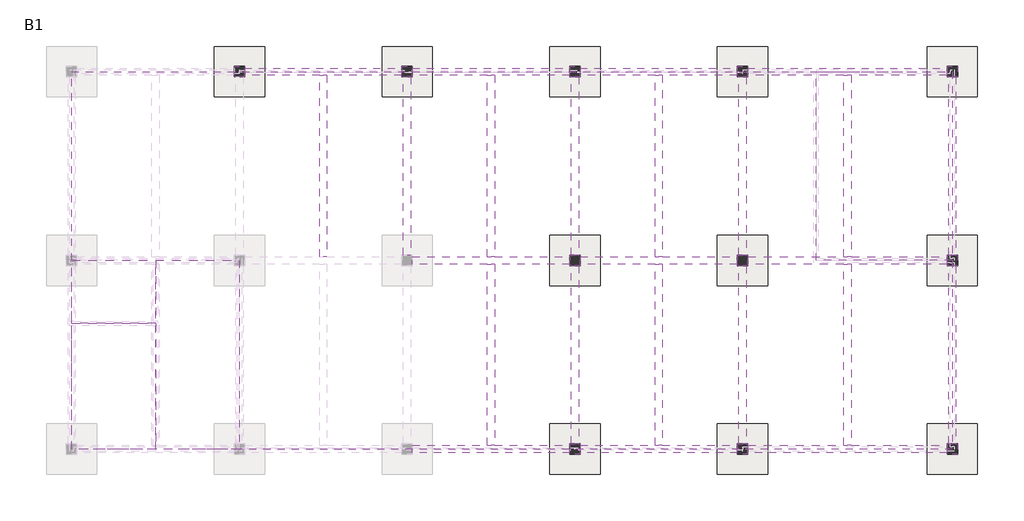
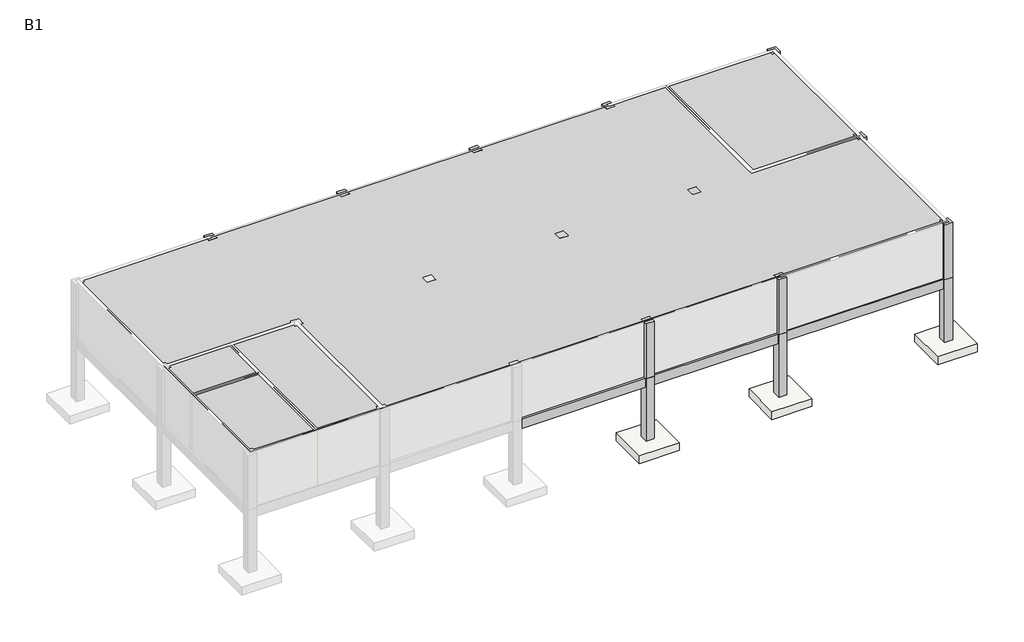
# One storey, part 2 of 2: 24 beams, 22 columns, 11 slabs, 5 proxies.
"""IFC4 building model written with IfcOpenShell, lengths in millimetres."""

import ifcopenshell
import ifcopenshell.guid

model = None  # the IFC model being written
_history = None  # IfcOwnerHistory: only IFC2X3 demands one
_inside = {}  # id of a spatial element -> (the spatial element, [elements in it])
_under = {}  # id of a project, library or spatial element -> (it, [spatial elements below it])
_declared = {}  # id of a project -> (the project, [libraries it declares])
_typed = {}  # id of a type object -> (the type object, [elements of that type])
_made_of = {}  # id of a material, layer set ... -> (it, [elements and type objects made of it])


def new_model(schema):
    """Start an empty IFC model of exactly this schema.

    Asked for "IFC4X3", IfcOpenShell would pick the latest addendum, in which some entities
    have other attributes; the version numbers below select the first issue.
    IFC2X3 requires an IfcOwnerHistory on every rooted entity: one is made here for all.
    """
    global model, _history
    if schema == "IFC4X3":
        model = ifcopenshell.file(schema_version=(4, 3, 0, 0))
    else:
        model = ifcopenshell.file(schema=schema)
    _inside.clear()
    _under.clear()
    _declared.clear()
    _typed.clear()
    _made_of.clear()
    _history = None
    if model.schema == "IFC2X3":
        org = make("IfcOrganization", Name="unknown")
        user = make(
            "IfcPersonAndOrganization",
            ThePerson=make("IfcPerson", FamilyName="unknown"),
            TheOrganization=org,
        )
        app = make(
            "IfcApplication",
            ApplicationDeveloper=org,
            Version="unknown",
            ApplicationFullName="unknown",
            ApplicationIdentifier="unknown",
        )
        _history = make(
            "IfcOwnerHistory",
            OwningUser=user,
            OwningApplication=app,
            ChangeAction="ADDED",
            CreationDate=0,
        )
    return model


def make(cls, **values):
    """One entity of the class cls with the attributes given. An attribute that is None is left unset."""
    return model.create_entity(
        cls, **{name: value for name, value in values.items() if value is not None}
    )


def rooted(cls, **values):
    """An entity with a GlobalId (a new one), such as an element, a storey or a relation."""
    return make(cls, GlobalId=ifcopenshell.guid.new(), OwnerHistory=_history, **values)


def si_unit(unit_type, name, prefix=None):
    """IfcSIUnit, for example si_unit("LENGTHUNIT", "METRE", prefix="MILLI")."""
    return make("IfcSIUnit", UnitType=unit_type, Prefix=prefix, Name=name)


def assignment(units):
    """IfcUnitAssignment: the units of a project."""
    return None if units is None else make("IfcUnitAssignment", Units=units)


def point(xyz):
    """IfcCartesianPoint."""
    return None if xyz is None else make("IfcCartesianPoint", Coordinates=xyz)


def direction(xyz):
    """IfcDirection."""
    return None if xyz is None else make("IfcDirection", DirectionRatios=xyz)


def frame(location, z_axis=None, x_axis=None):
    """IfcAxis2Placement3D, a coordinate frame: its origin and axes. An axis left out is left unset."""
    return make(
        "IfcAxis2Placement3D",
        Location=point(location),
        Axis=direction(z_axis),
        RefDirection=direction(x_axis),
    )


def origin():
    """The frame at (0, 0, 0) with its axes left unset."""
    return frame((0.0, 0.0, 0.0))


def origin_with_axes():
    """The frame at (0, 0, 0) with the z axis (0, 0, 1) and the x axis (1, 0, 0) written out."""
    return frame((0.0, 0.0, 0.0), z_axis=(0.0, 0.0, 1.0), x_axis=(1.0, 0.0, 0.0))


def place(relative_to, where):
    """IfcLocalPlacement: puts the frame where relative to a parent placement (None: the world)."""
    return make(
        "IfcLocalPlacement", PlacementRelTo=relative_to, RelativePlacement=where
    )


def context(
    kind, dimensions, precision=None, world=None, true_north=None, identifier=None
):
    """IfcGeometricRepresentationContext, for example the 3D "Model" context."""
    return make(
        "IfcGeometricRepresentationContext",
        ContextIdentifier=identifier,
        ContextType=kind,
        CoordinateSpaceDimension=dimensions,
        Precision=precision,
        WorldCoordinateSystem=world,
        TrueNorth=true_north,
    )


def project(units=None, contexts=None):
    """IfcProject with its units and contexts."""
    return rooted(
        "IfcProject",
        Name="project",
        RepresentationContexts=contexts,
        UnitsInContext=assignment(units),
    )


def spatial(cls, under=None, at=None, **own):
    """A site, building, storey or space (cls), placed at a placement, below another one or the project."""
    s = rooted(cls, ObjectPlacement=at, **own)
    if under is not None:
        _under.setdefault(under.id(), (under, []))[1].append(s)
    return s


def polyline(points):
    """IfcPolyline through the points."""
    return make("IfcPolyline", Points=[point(p) for p in points])


def outline(outer, holes=None, kind="AREA"):
    """IfcArbitraryClosedProfileDef: a profile drawn as a closed curve; with holes, ...WithVoids."""
    if holes is None:
        return make("IfcArbitraryClosedProfileDef", ProfileType=kind, OuterCurve=outer)
    return make(
        "IfcArbitraryProfileDefWithVoids",
        ProfileType=kind,
        OuterCurve=outer,
        InnerCurves=holes,
    )


def extrude(swept, where, along, depth):
    """IfcExtrudedAreaSolid: the profile swept, set in the frame where, extruded along a direction by depth."""
    return make(
        "IfcExtrudedAreaSolid",
        SweptArea=swept,
        Position=where,
        ExtrudedDirection=direction(along),
        Depth=depth,
    )


def faces_of(points, faces, orient=None, outer=None):
    """IfcFace entities. A face is a list of loops; a loop is a list of indices into points, from 0.

    orient and outer hold one flag for each loop. By default every Orientation is true, the
    first loop of a face is its IfcFaceOuterBound and the others are IfcFaceBound.
    """
    made = []
    for i, loops in enumerate(faces):
        bounds = []
        for j, loop in enumerate(loops):
            is_outer = j == 0 if outer is None else outer[i][j]
            bounds.append(
                make(
                    "IfcFaceOuterBound" if is_outer else "IfcFaceBound",
                    Bound=make("IfcPolyLoop", Polygon=[points[k] for k in loop]),
                    Orientation=True if orient is None else orient[i][j],
                )
            )
        made.append(make("IfcFace", Bounds=bounds))
    return made


def faceted_brep(points, faces, orient=None, outer=None, voids=None):
    """IfcFacetedBrep: a solid bounded by flat faces; with voids (closed shells), ...WithVoids."""
    shared = [point(p) for p in points]
    hull = make("IfcClosedShell", CfsFaces=faces_of(shared, faces, orient, outer))
    if voids is None:
        return make("IfcFacetedBrep", Outer=hull)
    return make(
        "IfcFacetedBrepWithVoids",
        Outer=hull,
        Voids=[
            make(cls, CfsFaces=faces_of(shared, fs, o, b)) for cls, fs, o, b in voids
        ],
    )


def shape(context_of_items, identifier, shape_type, items):
    """IfcShapeRepresentation: the items that make up one representation, for example the "Body"."""
    return make(
        "IfcShapeRepresentation",
        ContextOfItems=context_of_items,
        RepresentationIdentifier=identifier,
        RepresentationType=shape_type,
        Items=items,
    )


def source(mapping_origin, context_of_items, identifier, shape_type, items):
    """IfcRepresentationMap: a shape defined once, which mapped items show again and again."""
    return make(
        "IfcRepresentationMap",
        MappingOrigin=mapping_origin,
        MappedRepresentation=shape(context_of_items, identifier, shape_type, items),
    )


def transform(
    local_origin,
    x_axis=None,
    y_axis=None,
    z_axis=None,
    scale=None,
    scale2=None,
    scale3=None,
    uniform=True,
):
    """IfcCartesianTransformationOperator3D, or its non-uniform kind. x_axis, y_axis, z_axis: its Axis1, 2, 3."""
    if uniform:
        return make(
            "IfcCartesianTransformationOperator3D",
            Axis1=direction(x_axis),
            Axis2=direction(y_axis),
            LocalOrigin=point(local_origin),
            Scale=scale,
            Axis3=direction(z_axis),
        )
    return make(
        "IfcCartesianTransformationOperator3DnonUniform",
        Axis1=direction(x_axis),
        Axis2=direction(y_axis),
        LocalOrigin=point(local_origin),
        Scale=scale,
        Axis3=direction(z_axis),
        Scale2=scale2,
        Scale3=scale3,
    )


def mapped(mapping_source, mapping_target):
    """IfcMappedItem: shows the shape of a source again, moved by a transform."""
    return make(
        "IfcMappedItem", MappingSource=mapping_source, MappingTarget=mapping_target
    )


def made_of(thing, what):
    """Note that an element or type object is made of a material, layer set ...; save() writes the relation."""
    if what is not None:
        _made_of.setdefault(what.id(), (what, []))[1].append(thing)
    return thing


def element(
    cls,
    number,
    at=None,
    inside=None,
    cuts=None,
    type_object=None,
    material=None,
    context=None,
    identifier="Body",
    shape_type=None,
    held_by="IfcProductDefinitionShape",
    body=None,
    shapes=None,
    **own,
):
    """One element of the class cls, such as IfcWall. Its Tag is "e" and its number.

    at: its placement. inside: the storey or other place that contains it. cuts: it is an
    opening in that element (IfcRelVoidsElement). A single representation is given by context,
    identifier, shape_type and body (its items); several are given by shapes. held_by: the class
    of the entity that holds the representations. save() writes the other relations.
    """
    e = rooted(cls, Tag="e%d" % number, ObjectPlacement=at, **own)
    if body is not None:
        shapes = [shape(context, identifier, shape_type, body)]
    if shapes is not None:
        e.Representation = make(held_by, Representations=shapes)
    if inside is not None:
        _inside.setdefault(inside.id(), (inside, []))[1].append(e)
    if cuts is not None:
        rooted(
            "IfcRelVoidsElement", RelatingBuildingElement=cuts, RelatedOpeningElement=e
        )
    if type_object is not None:
        _typed.setdefault(type_object.id(), (type_object, []))[1].append(e)
    return made_of(e, material)


def aggregate(whole, parts):
    """IfcRelAggregates: a whole, such as a stair, and the parts it consists of."""
    return rooted("IfcRelAggregates", RelatingObject=whole, RelatedObjects=parts)


def save(model, path):
    """Write the relations noted so far, then the file.

    IfcRelAggregates (storeys below a building ...), IfcRelContainedInSpatialStructure (elements
    in a storey), IfcRelDefinesByType, IfcRelAssociatesMaterial and IfcRelDeclares: one each for
    every whole, place, type object, material and project.
    """
    for whole, parts in _under.values():
        aggregate(whole, parts)
    for where, things in _inside.values():
        rooted(
            "IfcRelContainedInSpatialStructure",
            RelatedElements=things,
            RelatingStructure=where,
        )
    for kind, things in _typed.values():
        rooted("IfcRelDefinesByType", RelatedObjects=things, RelatingType=kind)
    for what, things in _made_of.values():
        rooted("IfcRelAssociatesMaterial", RelatedObjects=things, RelatingMaterial=what)
    for by, libraries in _declared.values():
        rooted("IfcRelDeclares", RelatingContext=by, RelatedDefinitions=libraries)
    model.write(path)


def generic_models_bb515c93(model_context):
    return source(origin(), model_context, "Body", "SweptSolid", [
        extrude(outline(polyline([(9000.0, 21000.0), (9000.0, -21000.0), (-9000.0, -21000.0), (-9000.0, 21000.0), (9000.0, 21000.0)])), origin_with_axes(), (0.0, 0.0, 1.0), 3500.0),
    ])


def generic_models_5926095e(model_context):
    return source(origin(), model_context, "Body", "SweptSolid", [
        extrude(outline(polyline([(3250.0, 4500.0), (3250.0, -4500.0), (-3250.0, -4500.0), (-3250.0, 4500.0), (3250.0, 4500.0)])), origin_with_axes(), (0.0, 0.0, 1.0), 3500.0),
    ])


def generic_models_0b067365(model_context):
    return source(origin(), model_context, "Body", "SweptSolid", [
        extrude(outline(polyline([(2000.0, 4500.0), (2000.0, -4500.0), (-2000.0, -4500.0), (-2000.0, 4500.0), (2000.0, 4500.0)])), origin_with_axes(), (0.0, 0.0, 1.0), 3500.0),
    ])


def generic_models_4c644d41(model_context):
    return source(origin(), model_context, "Body", "SweptSolid", [
        extrude(outline(polyline([(2000.0, 1500.0), (2000.0, -1500.0), (-2000.0, -1500.0), (-2000.0, 1500.0), (2000.0, 1500.0)])), origin_with_axes(), (0.0, 0.0, 1.0), 3500.0),
    ])


def generic_models_c89eb543(model_context):
    return source(origin(), model_context, "Body", "SweptSolid", [
        extrude(outline(polyline([(2000.0, 3000.0), (2000.0, -3000.0), (-2000.0, -3000.0), (-2000.0, 3000.0), (2000.0, 3000.0)])), origin_with_axes(), (0.0, 0.0, 1.0), 3500.0),
    ])


def ft112_footing_rectangular_ft112_2400x2400x500_5fe39465(model_context):
    return source(origin(), model_context, "Body", "SweptSolid", [
        extrude(outline(polyline([(1200.0, 1200.0), (1200.0, -1200.0), (-1200.0, -1200.0), (-1200.0, 1200.0), (1200.0, 1200.0)])), frame((0.0, 0.0, -500.0), z_axis=(0.0, 0.0, 1.0), x_axis=(1.0, 0.0, 0.0)), (0.0, 0.0, 1.0), 500.0),
    ])


model = new_model("IFC4")

# Units and contexts
model_context = context("Model", 3, world=origin())
ifc_project = project(units=[si_unit("LENGTHUNIT", "METRE", prefix="MILLI")], contexts=[model_context])

# Site, building, storey
site = spatial("IfcSite", under=ifc_project)
building = spatial("IfcBuilding", under=site)
storey = spatial("IfcBuildingStorey", under=building, Name="B1", Elevation=-4000.0)

# Beams
placement = place(None, origin())
element("IfcBeam", 1, ObjectType="Concrete-Rectangular-Beam : BM111_400x500_RG1", at=placement, inside=storey, context=model_context, shape_type="SweptSolid", body=[
    extrude(outline(polyline([(57634.6521483, 173098.8614395), (57284.6521483, 173098.8614395), (57284.6521483, 181748.8614395), (57634.6521483, 181748.8614395), (57634.6521483, 173098.8614395)])), frame((0.0, 0.0, -600.0), z_axis=(0.0, 0.0, 1.0), x_axis=(1.0, 0.0, 0.0)), (0.0, 0.0, 1.0), 600.0),
])
element("IfcBeam", 2, ObjectType="Concrete-Rectangular-Beam : BM111_400x500_RG1", at=placement, inside=storey, context=model_context, shape_type="SweptSolid", body=[
    extrude(outline(polyline([(65634.6521483, 173098.8614395), (65284.6521483, 173098.8614395), (65284.6521483, 181748.8614395), (65634.6521483, 181748.8614395), (65634.6521483, 173098.8614395)])), frame((0.0, 0.0, -600.0), z_axis=(0.0, 0.0, 1.0), x_axis=(1.0, 0.0, 0.0)), (0.0, 0.0, 1.0), 600.0),
])
element("IfcBeam", 3, ObjectType="Concrete-Rectangular-Beam : BM111_400x500_RG1", at=placement, inside=storey, context=model_context, shape_type="SweptSolid", body=[
    extrude(outline(polyline([(65284.6521483, 172748.8614395), (65634.6521483, 172748.8614395), (65634.6521483, 164098.8614395), (65284.6521483, 164098.8614395), (65284.6521483, 172748.8614395)])), frame((0.0, 0.0, -600.0), z_axis=(0.0, 0.0, 1.0), x_axis=(1.0, 0.0, 0.0)), (0.0, 0.0, 1.0), 600.0),
])
element("IfcBeam", 4, ObjectType="Concrete-Rectangular-Beam : BM111_400x500_RG1", at=placement, inside=storey, context=model_context, shape_type="SweptSolid", body=[
    extrude(outline(polyline([(73634.6521483, 173098.8614395), (73284.6521483, 173098.8614395), (73284.6521483, 181748.8614395), (73634.6521483, 181748.8614395), (73634.6521483, 173098.8614395)])), frame((0.0, 0.0, -600.0), z_axis=(0.0, 0.0, 1.0), x_axis=(1.0, 0.0, 0.0)), (0.0, 0.0, 1.0), 600.0),
])
element("IfcBeam", 5, ObjectType="Concrete-Rectangular-Beam : BM111_400x500_RG1", at=placement, inside=storey, context=model_context, shape_type="SweptSolid", body=[
    extrude(outline(polyline([(73284.6521483, 172748.8614395), (73634.6521483, 172748.8614395), (73634.6521483, 164098.8614395), (73284.6521483, 164098.8614395), (73284.6521483, 172748.8614395)])), frame((0.0, 0.0, -600.0), z_axis=(0.0, 0.0, 1.0), x_axis=(1.0, 0.0, 0.0)), (0.0, 0.0, 1.0), 600.0),
])
element("IfcBeam", 6, ObjectType="Concrete-Rectangular-Beam : BM111_400x500_RG1", at=placement, inside=storey, context=model_context, shape_type="SweptSolid", body=[
    extrude(outline(polyline([(82634.6521483, 173098.8614395), (82284.6521483, 173098.8614395), (82284.6521483, 181748.8614395), (82634.6521483, 181748.8614395), (82634.6521483, 173098.8614395)])), frame((0.0, 0.0, -600.0), z_axis=(0.0, 0.0, 1.0), x_axis=(1.0, 0.0, 0.0)), (0.0, 0.0, 1.0), 600.0),
])
element("IfcBeam", 7, ObjectType="Concrete-Rectangular-Beam : BM111_400x500_RG1", at=placement, inside=storey, context=model_context, shape_type="SweptSolid", body=[
    extrude(outline(polyline([(82284.6521483, 172748.8614395), (82634.6521483, 172748.8614395), (82634.6521483, 164098.8614395), (82284.6521483, 164098.8614395), (82284.6521483, 172748.8614395)])), frame((0.0, 0.0, -600.0), z_axis=(0.0, 0.0, 1.0), x_axis=(1.0, 0.0, 0.0)), (0.0, 0.0, 1.0), 600.0),
])
element("IfcBeam", 8, ObjectType="Concrete-Rectangular-Beam : BM111_400x500_RG1", at=placement, inside=storey, context=model_context, shape_type="Brep", body=[
    faceted_brep([(53709.6521483, 182098.8614395, 0.0), (53709.6521483, 181748.8614395, 0.0), (57284.6521483, 181748.8614395, 0.0), (57634.6521483, 181748.8614395, 0.0), (61209.6521483, 181748.8614395, 0.0), (61209.6521483, 182098.8614395, 0.0), (53709.6521483, 181748.8614395, -600.0), (57284.6521483, 181748.8614395, -600.0), (57634.6521483, 181748.8614395, -600.0), (61209.6521483, 181748.8614395, -600.0), (53709.6521483, 182098.8614395, -600.0), (61209.6521483, 182098.8614395, -600.0)], [[[0, 1, 2, 3, 4, 5]], [[1, 6, 7, 8, 9, 4, 3, 2]], [[6, 10, 11, 9, 8, 7]], [[10, 0, 5, 11]], [[1, 0, 10, 6]], [[5, 4, 9, 11]]]),
])
element("IfcBeam", 9, ObjectType="Concrete-Rectangular-Beam : BM111_400x500_RG1", at=placement, inside=storey, context=model_context, shape_type="Brep", body=[
    faceted_brep([(61709.6521483, 182098.8614395, 0.0), (61709.6521483, 181748.8614395, 0.0), (65284.6521483, 181748.8614395, 0.0), (65634.6521483, 181748.8614395, 0.0), (69209.6521483, 181748.8614395, 0.0), (69209.6521483, 182098.8614395, 0.0), (61709.6521483, 181748.8614395, -600.0), (65284.6521483, 181748.8614395, -600.0), (65634.6521483, 181748.8614395, -600.0), (69209.6521483, 181748.8614395, -600.0), (61709.6521483, 182098.8614395, -600.0), (69209.6521483, 182098.8614395, -600.0)], [[[0, 1, 2, 3, 4, 5]], [[1, 6, 7, 8, 9, 4, 3, 2]], [[6, 10, 11, 9, 8, 7]], [[10, 0, 5, 11]], [[1, 0, 10, 6]], [[5, 4, 9, 11]]]),
])
element("IfcBeam", 10, ObjectType="Concrete-Rectangular-Beam : BM111_400x500_RG1", at=placement, inside=storey, context=model_context, shape_type="Brep", body=[
    faceted_brep([(69709.6521483, 182098.8614395, 0.0), (69709.6521483, 181748.8614395, 0.0), (73284.6521483, 181748.8614395, 0.0), (73634.6521483, 181748.8614395, 0.0), (77209.6521483, 181748.8614395, 0.0), (77209.6521483, 182098.8614395, 0.0), (69709.6521483, 181748.8614395, -600.0), (73284.6521483, 181748.8614395, -600.0), (73634.6521483, 181748.8614395, -600.0), (77209.6521483, 181748.8614395, -600.0), (69709.6521483, 182098.8614395, -600.0), (77209.6521483, 182098.8614395, -600.0)], [[[0, 1, 2, 3, 4, 5]], [[1, 6, 7, 8, 9, 4, 3, 2]], [[6, 10, 11, 9, 8, 7]], [[10, 0, 5, 11]], [[1, 0, 10, 6]], [[5, 4, 9, 11]]]),
])
element("IfcBeam", 11, ObjectType="Concrete-Rectangular-Beam : BM111_400x500_RG1", at=placement, inside=storey, context=model_context, shape_type="Brep", body=[
    faceted_brep([(77709.6521483, 182098.8614395, 0.0), (77709.6521483, 181748.8614395, 0.0), (82284.6521483, 181748.8614395, 0.0), (82634.6521483, 181748.8614395, 0.0), (87209.6521483, 181748.8614395, 0.0), (87209.6521483, 182098.8614395, 0.0), (77709.6521483, 181748.8614395, -600.0), (82284.6521483, 181748.8614395, -600.0), (82634.6521483, 181748.8614395, -600.0), (87209.6521483, 181748.8614395, -600.0), (77709.6521483, 182098.8614395, -600.0), (87209.6521483, 182098.8614395, -600.0)], [[[0, 1, 2, 3, 4, 5]], [[1, 6, 7, 8, 9, 4, 3, 2]], [[6, 10, 11, 9, 8, 7]], [[10, 0, 5, 11]], [[1, 0, 10, 6]], [[5, 4, 9, 11]]]),
])
element("IfcBeam", 12, ObjectType="Concrete-Rectangular-Beam : BM111_400x500_RG1", at=placement, inside=storey, context=model_context, shape_type="Brep", body=[
    faceted_brep([(61709.6521483, 173098.8614395, 0.0), (61709.6521483, 172748.8614395, 0.0), (65284.6521483, 172748.8614395, 0.0), (65634.6521483, 172748.8614395, 0.0), (69209.6521483, 172748.8614395, 0.0), (69209.6521483, 173098.8614395, 0.0), (65634.6521483, 173098.8614395, 0.0), (65284.6521483, 173098.8614395, 0.0), (61709.6521483, 172748.8614395, -600.0), (65284.6521483, 172748.8614395, -600.0), (65634.6521483, 172748.8614395, -600.0), (69209.6521483, 172748.8614395, -600.0), (61709.6521483, 173098.8614395, -600.0), (65284.6521483, 173098.8614395, -600.0), (65634.6521483, 173098.8614395, -600.0), (69209.6521483, 173098.8614395, -600.0)], [[[0, 1, 2, 3, 4, 5, 6, 7]], [[1, 8, 9, 10, 11, 4, 3, 2]], [[8, 12, 13, 14, 15, 11, 10, 9]], [[12, 0, 7, 6, 5, 15, 14, 13]], [[1, 0, 12, 8]], [[5, 4, 11, 15]]]),
])
element("IfcBeam", 13, ObjectType="Concrete-Rectangular-Beam : BM111_400x500_RG1", at=placement, inside=storey, context=model_context, shape_type="Brep", body=[
    faceted_brep([(69709.6521483, 173098.8614395, 0.0), (69709.6521483, 172748.8614395, 0.0), (73284.6521483, 172748.8614395, 0.0), (73634.6521483, 172748.8614395, 0.0), (77209.6521483, 172748.8614395, 0.0), (77209.6521483, 173098.8614395, 0.0), (73634.6521483, 173098.8614395, 0.0), (73284.6521483, 173098.8614395, 0.0), (69709.6521483, 172748.8614395, -600.0), (73284.6521483, 172748.8614395, -600.0), (73634.6521483, 172748.8614395, -600.0), (77209.6521483, 172748.8614395, -600.0), (69709.6521483, 173098.8614395, -600.0), (73284.6521483, 173098.8614395, -600.0), (73634.6521483, 173098.8614395, -600.0), (77209.6521483, 173098.8614395, -600.0)], [[[0, 1, 2, 3, 4, 5, 6, 7]], [[1, 8, 9, 10, 11, 4, 3, 2]], [[8, 12, 13, 14, 15, 11, 10, 9]], [[12, 0, 7, 6, 5, 15, 14, 13]], [[1, 0, 12, 8]], [[5, 4, 11, 15]]]),
])
element("IfcBeam", 14, ObjectType="Concrete-Rectangular-Beam : BM111_400x500_RG1", at=placement, inside=storey, context=model_context, shape_type="Brep", body=[
    faceted_brep([(77709.6521483, 173098.8614395, 0.0), (77709.6521483, 172748.8614395, 0.0), (82284.6521483, 172748.8614395, 0.0), (82634.6521483, 172748.8614395, 0.0), (87209.6521483, 172748.8614395, 0.0), (87209.6521483, 173098.8614395, 0.0), (82634.6521483, 173098.8614395, 0.0), (82284.6521483, 173098.8614395, 0.0), (77709.6521483, 172748.8614395, -600.0), (82284.6521483, 172748.8614395, -600.0), (82634.6521483, 172748.8614395, -600.0), (87209.6521483, 172748.8614395, -600.0), (77709.6521483, 173098.8614395, -600.0), (82284.6521483, 173098.8614395, -600.0), (82634.6521483, 173098.8614395, -600.0), (87209.6521483, 173098.8614395, -600.0)], [[[0, 1, 2, 3, 4, 5, 6, 7]], [[1, 8, 9, 10, 11, 4, 3, 2]], [[8, 12, 13, 14, 15, 11, 10, 9]], [[12, 0, 7, 6, 5, 15, 14, 13]], [[1, 0, 12, 8]], [[5, 4, 11, 15]]]),
])
element("IfcBeam", 15, ObjectType="Concrete-Rectangular-Beam : BM111_400x500_RG1", at=placement, inside=storey, context=model_context, shape_type="Brep", body=[
    faceted_brep([(61709.6521483, 164098.8614395, 0.0), (61709.6521483, 163748.8614395, 0.0), (69209.6521483, 163748.8614395, 0.0), (69209.6521483, 164098.8614395, 0.0), (65634.6521483, 164098.8614395, 0.0), (65284.6521483, 164098.8614395, 0.0), (61709.6521483, 163748.8614395, -600.0), (69209.6521483, 163748.8614395, -600.0), (61709.6521483, 164098.8614395, -600.0), (65284.6521483, 164098.8614395, -600.0), (65634.6521483, 164098.8614395, -600.0), (69209.6521483, 164098.8614395, -600.0)], [[[0, 1, 2, 3, 4, 5]], [[1, 6, 7, 2]], [[6, 8, 9, 10, 11, 7]], [[8, 0, 5, 4, 3, 11, 10, 9]], [[1, 0, 8, 6]], [[3, 2, 7, 11]]]),
])
element("IfcBeam", 16, ObjectType="Concrete-Rectangular-Beam : BM111_400x500_RG1", at=placement, inside=storey, context=model_context, shape_type="Brep", body=[
    faceted_brep([(69709.6521483, 164098.8614395, 0.0), (69709.6521483, 163748.8614395, 0.0), (77209.6521483, 163748.8614395, 0.0), (77209.6521483, 164098.8614395, 0.0), (73634.6521483, 164098.8614395, 0.0), (73284.6521483, 164098.8614395, 0.0), (69709.6521483, 163748.8614395, -600.0), (77209.6521483, 163748.8614395, -600.0), (69709.6521483, 164098.8614395, -600.0), (73284.6521483, 164098.8614395, -600.0), (73634.6521483, 164098.8614395, -600.0), (77209.6521483, 164098.8614395, -600.0)], [[[0, 1, 2, 3, 4, 5]], [[1, 6, 7, 2]], [[6, 8, 9, 10, 11, 7]], [[8, 0, 5, 4, 3, 11, 10, 9]], [[1, 0, 8, 6]], [[3, 2, 7, 11]]]),
])
element("IfcBeam", 17, ObjectType="Concrete-Rectangular-Beam : BM111_400x500_RG1", at=placement, inside=storey, context=model_context, shape_type="Brep", body=[
    faceted_brep([(77709.6521483, 164098.8614395, 0.0), (77709.6521483, 163748.8614395, 0.0), (87209.6521483, 163748.8614395, 0.0), (87209.6521483, 164098.8614395, 0.0), (82634.6521483, 164098.8614395, 0.0), (82284.6521483, 164098.8614395, 0.0), (77709.6521483, 163748.8614395, -600.0), (87209.6521483, 163748.8614395, -600.0), (77709.6521483, 164098.8614395, -600.0), (82284.6521483, 164098.8614395, -600.0), (82634.6521483, 164098.8614395, -600.0), (87209.6521483, 164098.8614395, -600.0)], [[[0, 1, 2, 3, 4, 5]], [[1, 6, 7, 2]], [[6, 8, 9, 10, 11, 7]], [[8, 0, 5, 4, 3, 11, 10, 9]], [[1, 0, 8, 6]], [[3, 2, 7, 11]]]),
])
element("IfcBeam", 18, ObjectType="Concrete-Rectangular-Beam : BM111_400x500_RG1", at=placement, inside=storey, context=model_context, shape_type="SweptSolid", body=[
    extrude(outline(polyline([(61284.6521483, 181673.8614395), (61634.6521483, 181673.8614395), (61634.6521483, 173173.8614395), (61284.6521483, 173173.8614395), (61284.6521483, 181673.8614395)])), frame((0.0, 0.0, -600.0), z_axis=(0.0, 0.0, 1.0), x_axis=(1.0, 0.0, 0.0)), (0.0, 0.0, 1.0), 600.0),
])
element("IfcBeam", 19, ObjectType="Concrete-Rectangular-Beam : BM111_400x500_RG1", at=placement, inside=storey, context=model_context, shape_type="SweptSolid", body=[
    extrude(outline(polyline([(69284.6521483, 181673.8614395), (69634.6521483, 181673.8614395), (69634.6521483, 173173.8614395), (69284.6521483, 173173.8614395), (69284.6521483, 181673.8614395)])), frame((0.0, 0.0, -600.0), z_axis=(0.0, 0.0, 1.0), x_axis=(1.0, 0.0, 0.0)), (0.0, 0.0, 1.0), 600.0),
])
element("IfcBeam", 20, ObjectType="Concrete-Rectangular-Beam : BM111_400x500_RG1", at=placement, inside=storey, context=model_context, shape_type="SweptSolid", body=[
    extrude(outline(polyline([(69284.6521483, 172673.8614395), (69634.6521483, 172673.8614395), (69634.6521483, 164173.8614395), (69284.6521483, 164173.8614395), (69284.6521483, 172673.8614395)])), frame((0.0, 0.0, -600.0), z_axis=(0.0, 0.0, 1.0), x_axis=(1.0, 0.0, 0.0)), (0.0, 0.0, 1.0), 600.0),
])
element("IfcBeam", 21, ObjectType="Concrete-Rectangular-Beam : BM111_400x500_RG1", at=placement, inside=storey, context=model_context, shape_type="SweptSolid", body=[
    extrude(outline(polyline([(77284.6521483, 181673.8614395), (77634.6521483, 181673.8614395), (77634.6521483, 173173.8614395), (77284.6521483, 173173.8614395), (77284.6521483, 181673.8614395)])), frame((0.0, 0.0, -600.0), z_axis=(0.0, 0.0, 1.0), x_axis=(1.0, 0.0, 0.0)), (0.0, 0.0, 1.0), 600.0),
])
element("IfcBeam", 22, ObjectType="Concrete-Rectangular-Beam : BM111_400x500_RG1", at=placement, inside=storey, context=model_context, shape_type="SweptSolid", body=[
    extrude(outline(polyline([(77284.6521483, 172673.8614395), (77634.6521483, 172673.8614395), (77634.6521483, 164173.8614395), (77284.6521483, 164173.8614395), (77284.6521483, 172673.8614395)])), frame((0.0, 0.0, -600.0), z_axis=(0.0, 0.0, 1.0), x_axis=(1.0, 0.0, 0.0)), (0.0, 0.0, 1.0), 600.0),
])
element("IfcBeam", 23, ObjectType="Concrete-Rectangular-Beam : BM111_400x500_RG1", at=placement, inside=storey, context=model_context, shape_type="SweptSolid", body=[
    extrude(outline(polyline([(87284.6521483, 181673.8614395), (87634.6521483, 181673.8614395), (87634.6521483, 173173.8614395), (87284.6521483, 173173.8614395), (87284.6521483, 181673.8614395)])), frame((0.0, 0.0, -600.0), z_axis=(0.0, 0.0, 1.0), x_axis=(1.0, 0.0, 0.0)), (0.0, 0.0, 1.0), 600.0),
])
element("IfcBeam", 24, ObjectType="Concrete-Rectangular-Beam : BM111_400x500_RG1", at=placement, inside=storey, context=model_context, shape_type="SweptSolid", body=[
    extrude(outline(polyline([(87284.6521483, 172673.8614395), (87634.6521483, 172673.8614395), (87634.6521483, 164173.8614395), (87284.6521483, 164173.8614395), (87284.6521483, 172673.8614395)])), frame((0.0, 0.0, -600.0), z_axis=(0.0, 0.0, 1.0), x_axis=(1.0, 0.0, 0.0)), (0.0, 0.0, 1.0), 600.0),
])

# Proxies
generic_models_shape = generic_models_bb515c93(model_context)
element("IfcBuildingElementProxy", 25, Name="Space Planning Box_hec : Space Planning Box_hec", ObjectType="Space Planning Box_hec : Space Planning Box_hec", at=placement, inside=storey, context=model_context, shape_type="MappedRepresentation", body=[
    mapped(generic_models_shape, transform((66459.6521483, 172923.8614395, 0.0), x_axis=(0.0, -1.0, 0.0), y_axis=(1.0, 0.0, 0.0), z_axis=(0.0, 0.0, 1.0))),
])
generic_models_2_shape = generic_models_5926095e(model_context)
element("IfcBuildingElementProxy", 26, Name="Space Planning Box_hec : Space Planning Box_hec", ObjectType="Space Planning Box_hec : Space Planning Box_hec", at=placement, inside=storey, context=model_context, shape_type="MappedRepresentation", body=[
    mapped(generic_models_2_shape, transform((84209.6521483, 177423.8614395, 0.0), x_axis=(1.0, 0.0, 0.0), y_axis=(0.0, 1.0, 0.0), z_axis=(0.0, 0.0, 1.0))),
])
generic_models_3_shape = generic_models_0b067365(model_context)
element("IfcBuildingElementProxy", 27, Name="Space Planning Box_hec : Space Planning Box_hec", ObjectType="Space Planning Box_hec : Space Planning Box_hec", at=placement, inside=storey, context=model_context, shape_type="MappedRepresentation", body=[
    mapped(generic_models_3_shape, transform((51459.6521483, 168423.8614395, 0.0), x_axis=(1.0, 0.0, 0.0), y_axis=(0.0, 1.0, 0.0), z_axis=(0.0, 0.0, 1.0))),
])
generic_models_4_shape = generic_models_4c644d41(model_context)
element("IfcBuildingElementProxy", 28, Name="Space Planning Box_hec : Space Planning Box_hec", ObjectType="Space Planning Box_hec : Space Planning Box_hec", at=placement, inside=storey, context=model_context, shape_type="MappedRepresentation", body=[
    mapped(generic_models_4_shape, transform((47459.6521483, 171423.8614395, 0.0), x_axis=(1.0, 0.0, 0.0), y_axis=(0.0, 1.0, 0.0), z_axis=(0.0, 0.0, 1.0))),
])
generic_models_5_shape = generic_models_c89eb543(model_context)
element("IfcBuildingElementProxy", 29, Name="Space Planning Box_hec : Space Planning Box_hec", ObjectType="Space Planning Box_hec : Space Planning Box_hec", at=placement, inside=storey, context=model_context, shape_type="MappedRepresentation", body=[
    mapped(generic_models_5_shape, transform((47459.6521483, 166923.8614395, 0.0), x_axis=(1.0, 0.0, 0.0), y_axis=(0.0, 1.0, 0.0), z_axis=(0.0, 0.0, 1.0))),
])

# Columns
element("IfcColumn", 30, ObjectType="Concrete-Rectangular-Column : CL111_500x500", at=placement, inside=storey, context=model_context, shape_type="Brep", body=[
    faceted_brep([(53709.6521483, 182173.8614395, 0.0), (53709.6521483, 181673.8614395, 0.0), (53209.6521483, 181673.8614395, 0.0), (53209.6521483, 182173.8614395, 0.0), (53709.6521483, 182173.8614395, 3500.0), (53709.6521483, 182098.8614395, 3500.0), (53709.6521483, 181748.8614395, 3500.0), (53709.6521483, 181673.8614395, 3500.0), (53634.6521483, 181673.8614395, 3500.0), (53284.6521483, 181673.8614395, 3500.0), (53209.6521483, 181673.8614395, 3500.0), (53209.6521483, 181748.8614395, 3500.0), (53209.6521483, 182098.8614395, 3500.0), (53209.6521483, 182173.8614395, 3500.0)], [[[0, 1, 2, 3]], [[4, 5, 6, 7, 1, 0]], [[7, 8, 9, 10, 2, 1]], [[10, 11, 12, 13, 3, 2]], [[13, 4, 0, 3]], [[4, 13, 12, 11, 10, 9, 8, 7, 6, 5]]]),
])
element("IfcColumn", 31, ObjectType="Concrete-Rectangular-Column : CL111_500x500", at=placement, inside=storey, context=model_context, shape_type="Brep", body=[
    faceted_brep([(61709.6521483, 182173.8614395, 0.0), (61709.6521483, 181673.8614395, 0.0), (61209.6521483, 181673.8614395, 0.0), (61209.6521483, 182173.8614395, 0.0), (61709.6521483, 182173.8614395, 3500.0), (61709.6521483, 182098.8614395, 3500.0), (61709.6521483, 181748.8614395, 3500.0), (61709.6521483, 181673.8614395, 3500.0), (61634.6521483, 181673.8614395, 3500.0), (61284.6521483, 181673.8614395, 3500.0), (61209.6521483, 181673.8614395, 3500.0), (61209.6521483, 181748.8614395, 3500.0), (61209.6521483, 182098.8614395, 3500.0), (61209.6521483, 182173.8614395, 3500.0)], [[[0, 1, 2, 3]], [[4, 5, 6, 7, 1, 0]], [[7, 8, 9, 10, 2, 1]], [[10, 11, 12, 13, 3, 2]], [[13, 4, 0, 3]], [[4, 13, 12, 11, 10, 9, 8, 7, 6, 5]]]),
])
element("IfcColumn", 32, ObjectType="Concrete-Rectangular-Column : CL111_500x500", at=placement, inside=storey, context=model_context, shape_type="Brep", body=[
    faceted_brep([(69709.6521483, 182173.8614395, 0.0), (69709.6521483, 181673.8614395, 0.0), (69209.6521483, 181673.8614395, 0.0), (69209.6521483, 182173.8614395, 0.0), (69709.6521483, 182173.8614395, 3500.0), (69709.6521483, 182098.8614395, 3500.0), (69709.6521483, 181748.8614395, 3500.0), (69709.6521483, 181673.8614395, 3500.0), (69634.6521483, 181673.8614395, 3500.0), (69284.6521483, 181673.8614395, 3500.0), (69209.6521483, 181673.8614395, 3500.0), (69209.6521483, 181748.8614395, 3500.0), (69209.6521483, 182098.8614395, 3500.0), (69209.6521483, 182173.8614395, 3500.0)], [[[0, 1, 2, 3]], [[4, 5, 6, 7, 1, 0]], [[7, 8, 9, 10, 2, 1]], [[10, 11, 12, 13, 3, 2]], [[13, 4, 0, 3]], [[4, 13, 12, 11, 10, 9, 8, 7, 6, 5]]]),
])
element("IfcColumn", 33, ObjectType="Concrete-Rectangular-Column : CL111_500x500", at=placement, inside=storey, context=model_context, shape_type="Brep", body=[
    faceted_brep([(77709.6521483, 182173.8614395, 0.0), (77709.6521483, 181673.8614395, 0.0), (77209.6521483, 181673.8614395, 0.0), (77209.6521483, 182173.8614395, 0.0), (77709.6521483, 182173.8614395, 3500.0), (77709.6521483, 182098.8614395, 3500.0), (77709.6521483, 181748.8614395, 3500.0), (77709.6521483, 181673.8614395, 3500.0), (77634.6521483, 181673.8614395, 3500.0), (77284.6521483, 181673.8614395, 3500.0), (77209.6521483, 181673.8614395, 3500.0), (77209.6521483, 181748.8614395, 3500.0), (77209.6521483, 182098.8614395, 3500.0), (77209.6521483, 182173.8614395, 3500.0)], [[[0, 1, 2, 3]], [[4, 5, 6, 7, 1, 0]], [[7, 8, 9, 10, 2, 1]], [[10, 11, 12, 13, 3, 2]], [[13, 4, 0, 3]], [[4, 13, 12, 11, 10, 9, 8, 7, 6, 5]]]),
])
element("IfcColumn", 34, ObjectType="Concrete-Rectangular-Column : CL111_500x500", at=placement, inside=storey, context=model_context, shape_type="Brep", body=[
    faceted_brep([(87709.6521483, 182173.8614395, 0.0), (87709.6521483, 181673.8614395, 0.0), (87209.6521483, 181673.8614395, 0.0), (87209.6521483, 182173.8614395, 0.0), (87709.6521483, 182173.8614395, 3500.0), (87709.6521483, 181673.8614395, 3500.0), (87634.6521483, 181673.8614395, 3500.0), (87284.6521483, 181673.8614395, 3500.0), (87209.6521483, 181673.8614395, 3500.0), (87209.6521483, 181748.8614395, 3500.0), (87209.6521483, 182098.8614395, 3500.0), (87209.6521483, 182173.8614395, 3500.0)], [[[0, 1, 2, 3]], [[4, 5, 1, 0]], [[5, 6, 7, 8, 2, 1]], [[8, 9, 10, 11, 3, 2]], [[11, 4, 0, 3]], [[4, 11, 10, 9, 8, 7, 6, 5]]]),
])
element("IfcColumn", 35, ObjectType="Concrete-Rectangular-Column : CL111_500x500", at=placement, inside=storey, context=model_context, shape_type="Brep", body=[
    faceted_brep([(69709.6521483, 173173.8614395, 0.0), (69709.6521483, 172673.8614395, 0.0), (69209.6521483, 172673.8614395, 0.0), (69209.6521483, 173173.8614395, 0.0), (69709.6521483, 173173.8614395, 3500.0), (69709.6521483, 173098.8614395, 3500.0), (69709.6521483, 172748.8614395, 3500.0), (69709.6521483, 172673.8614395, 3500.0), (69634.6521483, 172673.8614395, 3500.0), (69284.6521483, 172673.8614395, 3500.0), (69209.6521483, 172673.8614395, 3500.0), (69209.6521483, 172748.8614395, 3500.0), (69209.6521483, 173098.8614395, 3500.0), (69209.6521483, 173173.8614395, 3500.0), (69284.6521483, 173173.8614395, 3500.0), (69634.6521483, 173173.8614395, 3500.0)], [[[0, 1, 2, 3]], [[4, 5, 6, 7, 1, 0]], [[7, 8, 9, 10, 2, 1]], [[10, 11, 12, 13, 3, 2]], [[13, 14, 15, 4, 0, 3]], [[4, 15, 14, 13, 12, 11, 10, 9, 8, 7, 6, 5]]]),
])
element("IfcColumn", 36, ObjectType="Concrete-Rectangular-Column : CL111_500x500", at=placement, inside=storey, context=model_context, shape_type="Brep", body=[
    faceted_brep([(77709.6521483, 173173.8614395, 0.0), (77709.6521483, 172673.8614395, 0.0), (77209.6521483, 172673.8614395, 0.0), (77209.6521483, 173173.8614395, 0.0), (77709.6521483, 173173.8614395, 3500.0), (77709.6521483, 173098.8614395, 3500.0), (77709.6521483, 172748.8614395, 3500.0), (77709.6521483, 172673.8614395, 3500.0), (77634.6521483, 172673.8614395, 3500.0), (77284.6521483, 172673.8614395, 3500.0), (77209.6521483, 172673.8614395, 3500.0), (77209.6521483, 172748.8614395, 3500.0), (77209.6521483, 173098.8614395, 3500.0), (77209.6521483, 173173.8614395, 3500.0), (77284.6521483, 173173.8614395, 3500.0), (77634.6521483, 173173.8614395, 3500.0)], [[[0, 1, 2, 3]], [[4, 5, 6, 7, 1, 0]], [[7, 8, 9, 10, 2, 1]], [[10, 11, 12, 13, 3, 2]], [[13, 14, 15, 4, 0, 3]], [[4, 15, 14, 13, 12, 11, 10, 9, 8, 7, 6, 5]]]),
])
element("IfcColumn", 37, ObjectType="Concrete-Rectangular-Column : CL111_500x500", at=placement, inside=storey, context=model_context, shape_type="Brep", body=[
    faceted_brep([(87709.6521483, 173173.8614395, 0.0), (87709.6521483, 172673.8614395, 0.0), (87209.6521483, 172673.8614395, 0.0), (87209.6521483, 173173.8614395, 0.0), (87709.6521483, 173173.8614395, 3500.0), (87709.6521483, 172673.8614395, 3500.0), (87634.6521483, 172673.8614395, 3500.0), (87284.6521483, 172673.8614395, 3500.0), (87209.6521483, 172673.8614395, 3500.0), (87209.6521483, 172748.8614395, 3500.0), (87209.6521483, 173098.8614395, 3500.0), (87209.6521483, 173173.8614395, 3500.0), (87284.6521483, 173173.8614395, 3500.0), (87634.6521483, 173173.8614395, 3500.0)], [[[0, 1, 2, 3]], [[4, 5, 1, 0]], [[5, 6, 7, 8, 2, 1]], [[8, 9, 10, 11, 3, 2]], [[11, 12, 13, 4, 0, 3]], [[4, 13, 12, 11, 10, 9, 8, 7, 6, 5]]]),
])
element("IfcColumn", 38, ObjectType="Concrete-Rectangular-Column : CL111_500x500", at=placement, inside=storey, context=model_context, shape_type="Brep", body=[
    faceted_brep([(69709.6521483, 164173.8614395, 0.0), (69709.6521483, 163673.8614395, 0.0), (69209.6521483, 163673.8614395, 0.0), (69209.6521483, 164173.8614395, 0.0), (69709.6521483, 164173.8614395, 3500.0), (69709.6521483, 164098.8614395, 3500.0), (69709.6521483, 163748.8614395, 3500.0), (69709.6521483, 163673.8614395, 3500.0), (69209.6521483, 163673.8614395, 3500.0), (69209.6521483, 163748.8614395, 3500.0), (69209.6521483, 164098.8614395, 3500.0), (69209.6521483, 164173.8614395, 3500.0), (69284.6521483, 164173.8614395, 3500.0), (69634.6521483, 164173.8614395, 3500.0)], [[[0, 1, 2, 3]], [[4, 5, 6, 7, 1, 0]], [[7, 8, 2, 1]], [[8, 9, 10, 11, 3, 2]], [[11, 12, 13, 4, 0, 3]], [[4, 13, 12, 11, 10, 9, 8, 7, 6, 5]]]),
])
element("IfcColumn", 39, ObjectType="Concrete-Rectangular-Column : CL111_500x500", at=placement, inside=storey, context=model_context, shape_type="Brep", body=[
    faceted_brep([(77709.6521483, 164173.8614395, 0.0), (77709.6521483, 163673.8614395, 0.0), (77209.6521483, 163673.8614395, 0.0), (77209.6521483, 164173.8614395, 0.0), (77709.6521483, 164173.8614395, 3500.0), (77709.6521483, 164098.8614395, 3500.0), (77709.6521483, 163748.8614395, 3500.0), (77709.6521483, 163673.8614395, 3500.0), (77209.6521483, 163673.8614395, 3500.0), (77209.6521483, 163748.8614395, 3500.0), (77209.6521483, 164098.8614395, 3500.0), (77209.6521483, 164173.8614395, 3500.0), (77284.6521483, 164173.8614395, 3500.0), (77634.6521483, 164173.8614395, 3500.0)], [[[0, 1, 2, 3]], [[4, 5, 6, 7, 1, 0]], [[7, 8, 2, 1]], [[8, 9, 10, 11, 3, 2]], [[11, 12, 13, 4, 0, 3]], [[4, 13, 12, 11, 10, 9, 8, 7, 6, 5]]]),
])
element("IfcColumn", 40, ObjectType="Concrete-Rectangular-Column : CL111_500x500", at=placement, inside=storey, context=model_context, shape_type="Brep", body=[
    faceted_brep([(87709.6521483, 164173.8614395, 0.0), (87709.6521483, 163673.8614395, 0.0), (87209.6521483, 163673.8614395, 0.0), (87209.6521483, 164173.8614395, 0.0), (87709.6521483, 164173.8614395, 3500.0), (87709.6521483, 163673.8614395, 3500.0), (87209.6521483, 163673.8614395, 3500.0), (87209.6521483, 163748.8614395, 3500.0), (87209.6521483, 164098.8614395, 3500.0), (87209.6521483, 164173.8614395, 3500.0), (87284.6521483, 164173.8614395, 3500.0), (87634.6521483, 164173.8614395, 3500.0)], [[[0, 1, 2, 3]], [[4, 5, 1, 0]], [[5, 6, 2, 1]], [[6, 7, 8, 9, 3, 2]], [[9, 10, 11, 4, 0, 3]], [[4, 11, 10, 9, 8, 7, 6, 5]]]),
])
element("IfcColumn", 41, ObjectType="Concrete-Rectangular-Column : CL111_500x500", at=placement, inside=storey, context=model_context, shape_type="Brep", body=[
    faceted_brep([(53709.6521483, 182173.8614395, -4000.0), (53709.6521483, 181673.8614395, -4000.0), (53209.6521483, 181673.8614395, -4000.0), (53209.6521483, 182173.8614395, -4000.0), (53709.6521483, 182173.8614395, 0.0), (53709.6521483, 182098.8614395, 0.0), (53709.6521483, 181748.8614395, 0.0), (53709.6521483, 181673.8614395, 0.0), (53634.6521483, 181673.8614395, 0.0), (53284.6521483, 181673.8614395, 0.0), (53209.6521483, 181673.8614395, 0.0), (53209.6521483, 181748.8614395, 0.0), (53209.6521483, 182098.8614395, 0.0), (53209.6521483, 182173.8614395, 0.0)], [[[0, 1, 2, 3]], [[4, 5, 6, 7, 1, 0]], [[7, 8, 9, 10, 2, 1]], [[10, 11, 12, 13, 3, 2]], [[13, 4, 0, 3]], [[4, 13, 12, 11, 10, 9, 8, 7, 6, 5]]]),
])
element("IfcColumn", 42, ObjectType="Concrete-Rectangular-Column : CL111_500x500", at=placement, inside=storey, context=model_context, shape_type="Brep", body=[
    faceted_brep([(61709.6521483, 182173.8614395, -4000.0), (61709.6521483, 181673.8614395, -4000.0), (61209.6521483, 181673.8614395, -4000.0), (61209.6521483, 182173.8614395, -4000.0), (61709.6521483, 182173.8614395, 0.0), (61709.6521483, 182098.8614395, 0.0), (61709.6521483, 181748.8614395, 0.0), (61709.6521483, 181673.8614395, 0.0), (61634.6521483, 181673.8614395, 0.0), (61284.6521483, 181673.8614395, 0.0), (61209.6521483, 181673.8614395, 0.0), (61209.6521483, 181748.8614395, 0.0), (61209.6521483, 182098.8614395, 0.0), (61209.6521483, 182173.8614395, 0.0)], [[[0, 1, 2, 3]], [[4, 5, 6, 7, 1, 0]], [[7, 8, 9, 10, 2, 1]], [[10, 11, 12, 13, 3, 2]], [[13, 4, 0, 3]], [[4, 13, 12, 11, 10, 9, 8, 7, 6, 5]]]),
])
element("IfcColumn", 43, ObjectType="Concrete-Rectangular-Column : CL111_500x500", at=placement, inside=storey, context=model_context, shape_type="Brep", body=[
    faceted_brep([(69709.6521483, 182173.8614395, -4000.0), (69709.6521483, 181673.8614395, -4000.0), (69209.6521483, 181673.8614395, -4000.0), (69209.6521483, 182173.8614395, -4000.0), (69709.6521483, 182173.8614395, 0.0), (69709.6521483, 182098.8614395, 0.0), (69709.6521483, 181748.8614395, 0.0), (69709.6521483, 181673.8614395, 0.0), (69634.6521483, 181673.8614395, 0.0), (69284.6521483, 181673.8614395, 0.0), (69209.6521483, 181673.8614395, 0.0), (69209.6521483, 181748.8614395, 0.0), (69209.6521483, 182098.8614395, 0.0), (69209.6521483, 182173.8614395, 0.0)], [[[0, 1, 2, 3]], [[4, 5, 6, 7, 1, 0]], [[7, 8, 9, 10, 2, 1]], [[10, 11, 12, 13, 3, 2]], [[13, 4, 0, 3]], [[4, 13, 12, 11, 10, 9, 8, 7, 6, 5]]]),
])
element("IfcColumn", 44, ObjectType="Concrete-Rectangular-Column : CL111_500x500", at=placement, inside=storey, context=model_context, shape_type="Brep", body=[
    faceted_brep([(77709.6521483, 182173.8614395, -4000.0), (77709.6521483, 181673.8614395, -4000.0), (77209.6521483, 181673.8614395, -4000.0), (77209.6521483, 182173.8614395, -4000.0), (77709.6521483, 182173.8614395, 0.0), (77709.6521483, 182098.8614395, 0.0), (77709.6521483, 181748.8614395, 0.0), (77709.6521483, 181673.8614395, 0.0), (77634.6521483, 181673.8614395, 0.0), (77284.6521483, 181673.8614395, 0.0), (77209.6521483, 181673.8614395, 0.0), (77209.6521483, 181748.8614395, 0.0), (77209.6521483, 182098.8614395, 0.0), (77209.6521483, 182173.8614395, 0.0)], [[[0, 1, 2, 3]], [[4, 5, 6, 7, 1, 0]], [[7, 8, 9, 10, 2, 1]], [[10, 11, 12, 13, 3, 2]], [[13, 4, 0, 3]], [[4, 13, 12, 11, 10, 9, 8, 7, 6, 5]]]),
])
element("IfcColumn", 45, ObjectType="Concrete-Rectangular-Column : CL111_500x500", at=placement, inside=storey, context=model_context, shape_type="Brep", body=[
    faceted_brep([(87709.6521483, 182173.8614395, -4000.0), (87709.6521483, 181673.8614395, -4000.0), (87209.6521483, 181673.8614395, -4000.0), (87209.6521483, 182173.8614395, -4000.0), (87709.6521483, 182173.8614395, 0.0), (87709.6521483, 181673.8614395, 0.0), (87634.6521483, 181673.8614395, 0.0), (87284.6521483, 181673.8614395, 0.0), (87209.6521483, 181673.8614395, 0.0), (87209.6521483, 181748.8614395, 0.0), (87209.6521483, 182098.8614395, 0.0), (87209.6521483, 182173.8614395, 0.0)], [[[0, 1, 2, 3]], [[4, 5, 1, 0]], [[5, 6, 7, 8, 2, 1]], [[8, 9, 10, 11, 3, 2]], [[11, 4, 0, 3]], [[4, 11, 10, 9, 8, 7, 6, 5]]]),
])
element("IfcColumn", 46, ObjectType="Concrete-Rectangular-Column : CL111_500x500", at=placement, inside=storey, context=model_context, shape_type="Brep", body=[
    faceted_brep([(69709.6521483, 173173.8614395, -4000.0), (69709.6521483, 172673.8614395, -4000.0), (69209.6521483, 172673.8614395, -4000.0), (69209.6521483, 173173.8614395, -4000.0), (69709.6521483, 173173.8614395, 0.0), (69709.6521483, 173098.8614395, 0.0), (69709.6521483, 172748.8614395, 0.0), (69709.6521483, 172673.8614395, 0.0), (69634.6521483, 172673.8614395, 0.0), (69284.6521483, 172673.8614395, 0.0), (69209.6521483, 172673.8614395, 0.0), (69209.6521483, 172748.8614395, 0.0), (69209.6521483, 173098.8614395, 0.0), (69209.6521483, 173173.8614395, 0.0), (69284.6521483, 173173.8614395, 0.0), (69634.6521483, 173173.8614395, 0.0)], [[[0, 1, 2, 3]], [[4, 5, 6, 7, 1, 0]], [[7, 8, 9, 10, 2, 1]], [[10, 11, 12, 13, 3, 2]], [[13, 14, 15, 4, 0, 3]], [[4, 15, 14, 13, 12, 11, 10, 9, 8, 7, 6, 5]]]),
])
element("IfcColumn", 47, ObjectType="Concrete-Rectangular-Column : CL111_500x500", at=placement, inside=storey, context=model_context, shape_type="Brep", body=[
    faceted_brep([(77709.6521483, 173173.8614395, -4000.0), (77709.6521483, 172673.8614395, -4000.0), (77209.6521483, 172673.8614395, -4000.0), (77209.6521483, 173173.8614395, -4000.0), (77709.6521483, 173173.8614395, 0.0), (77709.6521483, 173098.8614395, 0.0), (77709.6521483, 172748.8614395, 0.0), (77709.6521483, 172673.8614395, 0.0), (77634.6521483, 172673.8614395, 0.0), (77284.6521483, 172673.8614395, 0.0), (77209.6521483, 172673.8614395, 0.0), (77209.6521483, 172748.8614395, 0.0), (77209.6521483, 173098.8614395, 0.0), (77209.6521483, 173173.8614395, 0.0), (77284.6521483, 173173.8614395, 0.0), (77634.6521483, 173173.8614395, 0.0)], [[[0, 1, 2, 3]], [[4, 5, 6, 7, 1, 0]], [[7, 8, 9, 10, 2, 1]], [[10, 11, 12, 13, 3, 2]], [[13, 14, 15, 4, 0, 3]], [[4, 15, 14, 13, 12, 11, 10, 9, 8, 7, 6, 5]]]),
])
element("IfcColumn", 48, ObjectType="Concrete-Rectangular-Column : CL111_500x500", at=placement, inside=storey, context=model_context, shape_type="Brep", body=[
    faceted_brep([(87709.6521483, 173173.8614395, -4000.0), (87709.6521483, 172673.8614395, -4000.0), (87209.6521483, 172673.8614395, -4000.0), (87209.6521483, 173173.8614395, -4000.0), (87709.6521483, 173173.8614395, 0.0), (87709.6521483, 172673.8614395, 0.0), (87634.6521483, 172673.8614395, 0.0), (87284.6521483, 172673.8614395, 0.0), (87209.6521483, 172673.8614395, 0.0), (87209.6521483, 172748.8614395, 0.0), (87209.6521483, 173098.8614395, 0.0), (87209.6521483, 173173.8614395, 0.0), (87284.6521483, 173173.8614395, 0.0), (87634.6521483, 173173.8614395, 0.0)], [[[0, 1, 2, 3]], [[4, 5, 1, 0]], [[5, 6, 7, 8, 2, 1]], [[8, 9, 10, 11, 3, 2]], [[11, 12, 13, 4, 0, 3]], [[4, 13, 12, 11, 10, 9, 8, 7, 6, 5]]]),
])
element("IfcColumn", 49, ObjectType="Concrete-Rectangular-Column : CL111_500x500", at=placement, inside=storey, context=model_context, shape_type="Brep", body=[
    faceted_brep([(69709.6521483, 164173.8614395, -4000.0), (69709.6521483, 163673.8614395, -4000.0), (69209.6521483, 163673.8614395, -4000.0), (69209.6521483, 164173.8614395, -4000.0), (69709.6521483, 164173.8614395, 0.0), (69709.6521483, 164098.8614395, 0.0), (69709.6521483, 163748.8614395, 0.0), (69709.6521483, 163673.8614395, 0.0), (69209.6521483, 163673.8614395, 0.0), (69209.6521483, 163748.8614395, 0.0), (69209.6521483, 164098.8614395, 0.0), (69209.6521483, 164173.8614395, 0.0), (69284.6521483, 164173.8614395, 0.0), (69634.6521483, 164173.8614395, 0.0)], [[[0, 1, 2, 3]], [[4, 5, 6, 7, 1, 0]], [[7, 8, 2, 1]], [[8, 9, 10, 11, 3, 2]], [[11, 12, 13, 4, 0, 3]], [[4, 13, 12, 11, 10, 9, 8, 7, 6, 5]]]),
])
element("IfcColumn", 50, ObjectType="Concrete-Rectangular-Column : CL111_500x500", at=placement, inside=storey, context=model_context, shape_type="Brep", body=[
    faceted_brep([(77709.6521483, 164173.8614395, -4000.0), (77709.6521483, 163673.8614395, -4000.0), (77209.6521483, 163673.8614395, -4000.0), (77209.6521483, 164173.8614395, -4000.0), (77709.6521483, 164173.8614395, 0.0), (77709.6521483, 164098.8614395, 0.0), (77709.6521483, 163748.8614395, 0.0), (77709.6521483, 163673.8614395, 0.0), (77209.6521483, 163673.8614395, 0.0), (77209.6521483, 163748.8614395, 0.0), (77209.6521483, 164098.8614395, 0.0), (77209.6521483, 164173.8614395, 0.0), (77284.6521483, 164173.8614395, 0.0), (77634.6521483, 164173.8614395, 0.0)], [[[0, 1, 2, 3]], [[4, 5, 6, 7, 1, 0]], [[7, 8, 2, 1]], [[8, 9, 10, 11, 3, 2]], [[11, 12, 13, 4, 0, 3]], [[4, 13, 12, 11, 10, 9, 8, 7, 6, 5]]]),
])
element("IfcColumn", 51, ObjectType="Concrete-Rectangular-Column : CL111_500x500", at=placement, inside=storey, context=model_context, shape_type="Brep", body=[
    faceted_brep([(87709.6521483, 164173.8614395, -4000.0), (87709.6521483, 163673.8614395, -4000.0), (87209.6521483, 163673.8614395, -4000.0), (87209.6521483, 164173.8614395, -4000.0), (87709.6521483, 164173.8614395, 0.0), (87709.6521483, 163673.8614395, 0.0), (87209.6521483, 163673.8614395, 0.0), (87209.6521483, 163748.8614395, 0.0), (87209.6521483, 164098.8614395, 0.0), (87209.6521483, 164173.8614395, 0.0), (87284.6521483, 164173.8614395, 0.0), (87634.6521483, 164173.8614395, 0.0)], [[[0, 1, 2, 3]], [[4, 5, 1, 0]], [[5, 6, 2, 1]], [[6, 7, 8, 9, 3, 2]], [[9, 10, 11, 4, 0, 3]], [[4, 11, 10, 9, 8, 7, 6, 5]]]),
])

# Slabs
ft112_footing_rectangular_ft112_2400x2400x500_shape = ft112_footing_rectangular_ft112_2400x2400x500_5fe39465(model_context)
element("IfcSlab", 52, ObjectType="FT112-Footing-Rectangular : FT112_2400x2400x500", at=placement, inside=storey, context=model_context, shape_type="MappedRepresentation", body=[
    mapped(ft112_footing_rectangular_ft112_2400x2400x500_shape, transform((53459.6521483, 181923.8614395, -4000.0), x_axis=(1.0, 0.0, 0.0), y_axis=(0.0, 1.0, 0.0), z_axis=(0.0, 0.0, 1.0))),
])
element("IfcSlab", 53, ObjectType="FT112-Footing-Rectangular : FT112_2400x2400x500", at=placement, inside=storey, context=model_context, shape_type="MappedRepresentation", body=[
    mapped(ft112_footing_rectangular_ft112_2400x2400x500_shape, transform((61459.6521483, 181923.8614395, -4000.0), x_axis=(1.0, 0.0, 0.0), y_axis=(0.0, 1.0, 0.0), z_axis=(0.0, 0.0, 1.0))),
])
element("IfcSlab", 54, ObjectType="FT112-Footing-Rectangular : FT112_2400x2400x500", at=placement, inside=storey, context=model_context, shape_type="MappedRepresentation", body=[
    mapped(ft112_footing_rectangular_ft112_2400x2400x500_shape, transform((69459.6521483, 181923.8614395, -4000.0), x_axis=(1.0, 0.0, 0.0), y_axis=(0.0, 1.0, 0.0), z_axis=(0.0, 0.0, 1.0))),
])
element("IfcSlab", 55, ObjectType="FT112-Footing-Rectangular : FT112_2400x2400x500", at=placement, inside=storey, context=model_context, shape_type="MappedRepresentation", body=[
    mapped(ft112_footing_rectangular_ft112_2400x2400x500_shape, transform((77459.6521483, 181923.8614395, -4000.0), x_axis=(1.0, 0.0, 0.0), y_axis=(0.0, 1.0, 0.0), z_axis=(0.0, 0.0, 1.0))),
])
element("IfcSlab", 56, ObjectType="FT112-Footing-Rectangular : FT112_2400x2400x500", at=placement, inside=storey, context=model_context, shape_type="MappedRepresentation", body=[
    mapped(ft112_footing_rectangular_ft112_2400x2400x500_shape, transform((87459.6521483, 181923.8614395, -4000.0), x_axis=(1.0, 0.0, 0.0), y_axis=(0.0, 1.0, 0.0), z_axis=(0.0, 0.0, 1.0))),
])
element("IfcSlab", 57, ObjectType="FT112-Footing-Rectangular : FT112_2400x2400x500", at=placement, inside=storey, context=model_context, shape_type="MappedRepresentation", body=[
    mapped(ft112_footing_rectangular_ft112_2400x2400x500_shape, transform((69459.6521483, 172923.8614395, -4000.0), x_axis=(1.0, 0.0, 0.0), y_axis=(0.0, 1.0, 0.0), z_axis=(0.0, 0.0, 1.0))),
])
element("IfcSlab", 58, ObjectType="FT112-Footing-Rectangular : FT112_2400x2400x500", at=placement, inside=storey, context=model_context, shape_type="MappedRepresentation", body=[
    mapped(ft112_footing_rectangular_ft112_2400x2400x500_shape, transform((77459.6521483, 172923.8614395, -4000.0), x_axis=(1.0, 0.0, 0.0), y_axis=(0.0, 1.0, 0.0), z_axis=(0.0, 0.0, 1.0))),
])
element("IfcSlab", 59, ObjectType="FT112-Footing-Rectangular : FT112_2400x2400x500", at=placement, inside=storey, context=model_context, shape_type="MappedRepresentation", body=[
    mapped(ft112_footing_rectangular_ft112_2400x2400x500_shape, transform((87459.6521483, 172923.8614395, -4000.0), x_axis=(1.0, 0.0, 0.0), y_axis=(0.0, 1.0, 0.0), z_axis=(0.0, 0.0, 1.0))),
])
element("IfcSlab", 60, ObjectType="FT112-Footing-Rectangular : FT112_2400x2400x500", at=placement, inside=storey, context=model_context, shape_type="MappedRepresentation", body=[
    mapped(ft112_footing_rectangular_ft112_2400x2400x500_shape, transform((69459.6521483, 163923.8614395, -4000.0), x_axis=(1.0, 0.0, 0.0), y_axis=(0.0, 1.0, 0.0), z_axis=(0.0, 0.0, 1.0))),
])
element("IfcSlab", 61, ObjectType="FT112-Footing-Rectangular : FT112_2400x2400x500", at=placement, inside=storey, context=model_context, shape_type="MappedRepresentation", body=[
    mapped(ft112_footing_rectangular_ft112_2400x2400x500_shape, transform((77459.6521483, 163923.8614395, -4000.0), x_axis=(1.0, 0.0, 0.0), y_axis=(0.0, 1.0, 0.0), z_axis=(0.0, 0.0, 1.0))),
])
element("IfcSlab", 62, ObjectType="FT112-Footing-Rectangular : FT112_2400x2400x500", at=placement, inside=storey, context=model_context, shape_type="MappedRepresentation", body=[
    mapped(ft112_footing_rectangular_ft112_2400x2400x500_shape, transform((87459.6521483, 163923.8614395, -4000.0), x_axis=(1.0, 0.0, 0.0), y_axis=(0.0, 1.0, 0.0), z_axis=(0.0, 0.0, 1.0))),
])

save(model, "model.ifc")

# Revit data of these elements
# Type "Concrete-Rectangular-Beam : BM111_400x500_RG1"
#   중앙부 하부근 = "3-D20"
#   중앙부 상부근 = "3-D20"
#   중앙부 보조근 = ""
#   중앙부 늑근 = "2-D10 @200"
#   외단부 하부근 = "3-D20"
#   외단부 상부근 = "3-D20"
#   외단부 보조근 = ""
#   외단부 늑근 = "2-D10 @100"
#   부호 = "RG1"
#   내단부 하부근 = "3-D20"
#   내단부 상부근 = "3-D20"
#   내단부 보조근 = ""
#   내단부 늑근 = "2-D10 @100"
#   ALL 하부근 = ""
#   ALL 상부근 = ""
#   ALL 보조근 = ""
#   ALL 늑근 = ""
#   Width = 400 mm
#   Height = 500 mm
#   Length [instance default] = 1524 mm
#   Structural Material [instance default] = 콘크리트 - 현장타설 콘크리트
#   hec_material3 [instance default] = none
#   hec_material2 [instance default] = none
#   hec_material1 [instance default] = none
#   Assembly Code = ""
# Type "Space Planning Box_hec : Space Planning Box_hec"
#   Type Comments = "..."
#   Room Name [instance default] = "?"
#   Interior Finish [instance default] = ""
#   Exterior Finish [instance default] = ""
#   Department [instance default] = ""
#   Assembly Code = "..."
#   ceiling height [instance default] = 0
#   Width [instance default] = 1524 mm
#   Program Area [instance default] = 0.00 m²
#   Length [instance default] = 1524 mm
#   Height [instance default] = 1524 mm
#   Area [instance default] = 2.32258 m²
#   Fill Color [instance default] = Cyan
#   Default Elevation = 0
# Type "Concrete-Rectangular-Column : CL111_500x500"
#   Description = "UG 철골 기둥용 Pedestal"
#   b = 500 mm
#   h = 500 mm
#   hec_material3 [instance default] = none
#   hec_material2 [instance default] = A03AE056-00001_Bitumen/Bituminous/Asphalt Coating
#   hec_material1 [instance default] = A03AC035-00001_Form Work (3 times in use)_Flat
#   Structural Material [instance default] = A03AC032-00007_Structural Concrete_Type1_25MPa-30Mpa
# Type "FT112-Footing-Rectangular : FT112_2400x2400x500"
#   Description = "UG Shallow Foundation"
#   Width = 2400 mm
#   Length = 2400 mm
#   Foundation Thickness = 500 mm
#   hec_material3 [instance default] = none
#   hec_material2 [instance default] = A03AE056-00001_Bitumen/Bituminous/Asphalt Coating
#   hec_material1 [instance default] = A03AC035-00001_Form Work (3 times in use)_Flat
#   Structural Material [instance default] = A03AC032-00007_Structural Concrete_Type1_25MPa-30Mpa
#   Assembly Code = ""
# Elements 1, 2, 3, 4, 5, 6, 7, 8, 9, 10, 11, 12, 13, 14, 15, 16, 17, 18, 19, 20, 21, 22, 23, 24 (IfcBeam, "Concrete-Rectangular-Beam : BM111_400x500_RG1")
#   Comments = ""
#   hec_material3 = none
#   hec_material2 = none
#   hec_material1 = none
#   Structural Material = 콘크리트 - 현장타설 콘크리트
#   Phase Created = New Construction
#   Materials on its faces: "콘크리트 - 현장타설 콘크리트"
# Element 25 (IfcBuildingElementProxy, "Space Planning Box_hec : Space Planning Box_hec")
#   Room Name = "Cable Room"
#   Interior Finish = "IW5..IW2..N/A,,WK1..N/A,,FL1..N/A,,CL1..N/A"
